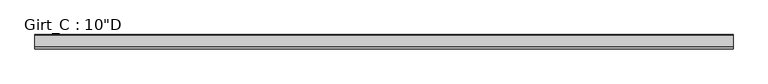
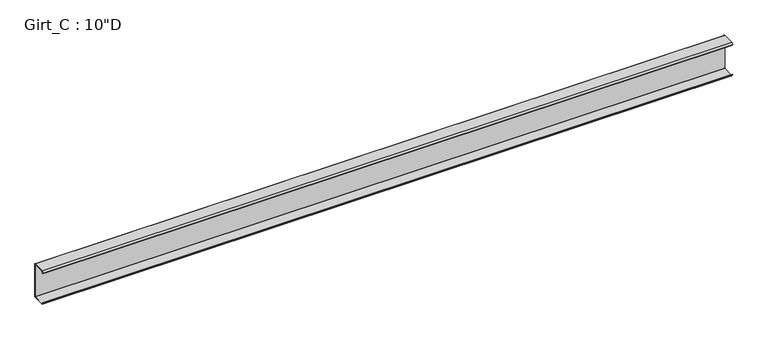
"""IFC4 building model written with IfcOpenShell, lengths in millimetres: beam geometry."""

import ifcopenshell
import ifcopenshell.guid

model = None  # the IFC model being written
_history = None  # IfcOwnerHistory: only IFC2X3 demands one
_inside = {}  # id of a spatial element -> (the spatial element, [elements in it])
_under = {}  # id of a project, library or spatial element -> (it, [spatial elements below it])
_declared = {}  # id of a project -> (the project, [libraries it declares])
_typed = {}  # id of a type object -> (the type object, [elements of that type])
_made_of = {}  # id of a material, layer set ... -> (it, [elements and type objects made of it])


def new_model(schema):
    """Start an empty IFC model of exactly this schema.

    Asked for "IFC4X3", IfcOpenShell would pick the latest addendum, in which some entities
    have other attributes; the version numbers below select the first issue.
    IFC2X3 requires an IfcOwnerHistory on every rooted entity: one is made here for all.
    """
    global model, _history
    if schema == "IFC4X3":
        model = ifcopenshell.file(schema_version=(4, 3, 0, 0))
    else:
        model = ifcopenshell.file(schema=schema)
    _inside.clear()
    _under.clear()
    _declared.clear()
    _typed.clear()
    _made_of.clear()
    _history = None
    if model.schema == "IFC2X3":
        org = make("IfcOrganization", Name="unknown")
        user = make(
            "IfcPersonAndOrganization",
            ThePerson=make("IfcPerson", FamilyName="unknown"),
            TheOrganization=org,
        )
        app = make(
            "IfcApplication",
            ApplicationDeveloper=org,
            Version="unknown",
            ApplicationFullName="unknown",
            ApplicationIdentifier="unknown",
        )
        _history = make(
            "IfcOwnerHistory",
            OwningUser=user,
            OwningApplication=app,
            ChangeAction="ADDED",
            CreationDate=0,
        )
    return model


def make(cls, **values):
    """One entity of the class cls with the attributes given. An attribute that is None is left unset."""
    return model.create_entity(
        cls, **{name: value for name, value in values.items() if value is not None}
    )


def rooted(cls, **values):
    """An entity with a GlobalId (a new one), such as an element, a storey or a relation."""
    return make(cls, GlobalId=ifcopenshell.guid.new(), OwnerHistory=_history, **values)


def si_unit(unit_type, name, prefix=None):
    """IfcSIUnit, for example si_unit("LENGTHUNIT", "METRE", prefix="MILLI")."""
    return make("IfcSIUnit", UnitType=unit_type, Prefix=prefix, Name=name)


def assignment(units):
    """IfcUnitAssignment: the units of a project."""
    return None if units is None else make("IfcUnitAssignment", Units=units)


def point(xyz):
    """IfcCartesianPoint."""
    return None if xyz is None else make("IfcCartesianPoint", Coordinates=xyz)


def direction(xyz):
    """IfcDirection."""
    return None if xyz is None else make("IfcDirection", DirectionRatios=xyz)


def frame(location, z_axis=None, x_axis=None):
    """IfcAxis2Placement3D, a coordinate frame: its origin and axes. An axis left out is left unset."""
    return make(
        "IfcAxis2Placement3D",
        Location=point(location),
        Axis=direction(z_axis),
        RefDirection=direction(x_axis),
    )


def frame_2d(location, x_axis=None):
    """IfcAxis2Placement2D, a coordinate frame in the plane: its origin and x axis."""
    return make(
        "IfcAxis2Placement2D", Location=point(location), RefDirection=direction(x_axis)
    )


def origin():
    """The frame at (0, 0, 0) with its axes left unset."""
    return frame((0.0, 0.0, 0.0))


def place(relative_to, where):
    """IfcLocalPlacement: puts the frame where relative to a parent placement (None: the world)."""
    return make(
        "IfcLocalPlacement", PlacementRelTo=relative_to, RelativePlacement=where
    )


def context(
    kind, dimensions, precision=None, world=None, true_north=None, identifier=None
):
    """IfcGeometricRepresentationContext, for example the 3D "Model" context."""
    return make(
        "IfcGeometricRepresentationContext",
        ContextIdentifier=identifier,
        ContextType=kind,
        CoordinateSpaceDimension=dimensions,
        Precision=precision,
        WorldCoordinateSystem=world,
        TrueNorth=true_north,
    )


def project(units=None, contexts=None):
    """IfcProject with its units and contexts."""
    return rooted(
        "IfcProject",
        Name="project",
        RepresentationContexts=contexts,
        UnitsInContext=assignment(units),
    )


def spatial(cls, under=None, at=None, **own):
    """A site, building, storey or space (cls), placed at a placement, below another one or the project."""
    s = rooted(cls, ObjectPlacement=at, **own)
    if under is not None:
        _under.setdefault(under.id(), (under, []))[1].append(s)
    return s


def polyline(points):
    """IfcPolyline through the points."""
    return make("IfcPolyline", Points=[point(p) for p in points])


def circle_curve(where, radius):
    """IfcCircle in the frame where."""
    return make("IfcCircle", Position=where, Radius=radius)


def trimmed(basis, trim1, trim2, sense, master):
    """IfcTrimmedCurve: the piece of a basis curve between two trims."""
    return make(
        "IfcTrimmedCurve",
        BasisCurve=basis,
        Trim1=trim1,
        Trim2=trim2,
        SenseAgreement=sense,
        MasterRepresentation=master,
    )


def segment(curve, same_sense, transition):
    """IfcCompositeCurveSegment."""
    return make(
        "IfcCompositeCurveSegment",
        Transition=transition,
        SameSense=same_sense,
        ParentCurve=curve,
    )


def composite_curve(segments, self_intersect=None):
    """IfcCompositeCurve: segments joined end to end."""
    return make("IfcCompositeCurve", Segments=segments, SelfIntersect=self_intersect)


def outline(outer, holes=None, kind="AREA"):
    """IfcArbitraryClosedProfileDef: a profile drawn as a closed curve; with holes, ...WithVoids."""
    if holes is None:
        return make("IfcArbitraryClosedProfileDef", ProfileType=kind, OuterCurve=outer)
    return make(
        "IfcArbitraryProfileDefWithVoids",
        ProfileType=kind,
        OuterCurve=outer,
        InnerCurves=holes,
    )


def extrude(swept, where, along, depth):
    """IfcExtrudedAreaSolid: the profile swept, set in the frame where, extruded along a direction by depth."""
    return make(
        "IfcExtrudedAreaSolid",
        SweptArea=swept,
        Position=where,
        ExtrudedDirection=direction(along),
        Depth=depth,
    )


def shape(context_of_items, identifier, shape_type, items):
    """IfcShapeRepresentation: the items that make up one representation, for example the "Body"."""
    return make(
        "IfcShapeRepresentation",
        ContextOfItems=context_of_items,
        RepresentationIdentifier=identifier,
        RepresentationType=shape_type,
        Items=items,
    )


def source(mapping_origin, context_of_items, identifier, shape_type, items):
    """IfcRepresentationMap: a shape defined once, which mapped items show again and again."""
    return make(
        "IfcRepresentationMap",
        MappingOrigin=mapping_origin,
        MappedRepresentation=shape(context_of_items, identifier, shape_type, items),
    )


def transform(
    local_origin,
    x_axis=None,
    y_axis=None,
    z_axis=None,
    scale=None,
    scale2=None,
    scale3=None,
    uniform=True,
):
    """IfcCartesianTransformationOperator3D, or its non-uniform kind. x_axis, y_axis, z_axis: its Axis1, 2, 3."""
    if uniform:
        return make(
            "IfcCartesianTransformationOperator3D",
            Axis1=direction(x_axis),
            Axis2=direction(y_axis),
            LocalOrigin=point(local_origin),
            Scale=scale,
            Axis3=direction(z_axis),
        )
    return make(
        "IfcCartesianTransformationOperator3DnonUniform",
        Axis1=direction(x_axis),
        Axis2=direction(y_axis),
        LocalOrigin=point(local_origin),
        Scale=scale,
        Axis3=direction(z_axis),
        Scale2=scale2,
        Scale3=scale3,
    )


def mapped(mapping_source, mapping_target):
    """IfcMappedItem: shows the shape of a source again, moved by a transform."""
    return make(
        "IfcMappedItem", MappingSource=mapping_source, MappingTarget=mapping_target
    )


def made_of(thing, what):
    """Note that an element or type object is made of a material, layer set ...; save() writes the relation."""
    if what is not None:
        _made_of.setdefault(what.id(), (what, []))[1].append(thing)
    return thing


def element(
    cls,
    number,
    at=None,
    inside=None,
    cuts=None,
    type_object=None,
    material=None,
    context=None,
    identifier="Body",
    shape_type=None,
    held_by="IfcProductDefinitionShape",
    body=None,
    shapes=None,
    **own,
):
    """One element of the class cls, such as IfcWall. Its Tag is "e" and its number.

    at: its placement. inside: the storey or other place that contains it. cuts: it is an
    opening in that element (IfcRelVoidsElement). A single representation is given by context,
    identifier, shape_type and body (its items); several are given by shapes. held_by: the class
    of the entity that holds the representations. save() writes the other relations.
    """
    e = rooted(cls, Tag="e%d" % number, ObjectPlacement=at, **own)
    if body is not None:
        shapes = [shape(context, identifier, shape_type, body)]
    if shapes is not None:
        e.Representation = make(held_by, Representations=shapes)
    if inside is not None:
        _inside.setdefault(inside.id(), (inside, []))[1].append(e)
    if cuts is not None:
        rooted(
            "IfcRelVoidsElement", RelatingBuildingElement=cuts, RelatedOpeningElement=e
        )
    if type_object is not None:
        _typed.setdefault(type_object.id(), (type_object, []))[1].append(e)
    return made_of(e, material)


def aggregate(whole, parts):
    """IfcRelAggregates: a whole, such as a stair, and the parts it consists of."""
    return rooted("IfcRelAggregates", RelatingObject=whole, RelatedObjects=parts)


def save(model, path):
    """Write the relations noted so far, then the file.

    IfcRelAggregates (storeys below a building ...), IfcRelContainedInSpatialStructure (elements
    in a storey), IfcRelDefinesByType, IfcRelAssociatesMaterial and IfcRelDeclares: one each for
    every whole, place, type object, material and project.
    """
    for whole, parts in _under.values():
        aggregate(whole, parts)
    for where, things in _inside.values():
        rooted(
            "IfcRelContainedInSpatialStructure",
            RelatedElements=things,
            RelatingStructure=where,
        )
    for kind, things in _typed.values():
        rooted("IfcRelDefinesByType", RelatedObjects=things, RelatingType=kind)
    for what, things in _made_of.values():
        rooted("IfcRelAssociatesMaterial", RelatedObjects=things, RelatingMaterial=what)
    for by, libraries in _declared.values():
        rooted("IfcRelDeclares", RelatingContext=by, RelatedDefinitions=libraries)
    model.write(path)


def beam_7096158d(model_context):
    return source(origin(), model_context, "Body", "SweptSolid", [
        extrude(outline(composite_curve([segment(polyline([(-87.5109375, 127.0), (-3.3734375, 127.0)]), True, "CONTINUOUS"), segment(trimmed(circle_curve(frame_2d((-3.3734375, 122.2375)), 4.7625), [point((-3.3734375, 127.0))], [point((1.3890625, 122.2375))], False, "CARTESIAN"), True, "CONTINUOUS"), segment(polyline([(1.3890625, 122.2375), (1.3890625, -122.2375)]), True, "CONTINUOUS"), segment(trimmed(circle_curve(frame_2d((-3.3734375, -122.2375)), 4.7625), [point((1.3890625, -122.2375))], [point((-3.3734375, -127.0))], False, "CARTESIAN"), True, "CONTINUOUS"), segment(polyline([(-3.3734375, -127.0), (-87.5109375, -127.0), (-99.7792647, -112.379177), (-97.6510975, -110.5934327), (-86.2154765, -124.221875), (-3.2694106, -124.221875)]), True, "CONTINUOUS"), segment(trimmed(circle_curve(frame_2d((-3.3748024, -122.2389339)), 1.9857399), [point((-3.2694106, -124.221875))], [point((-1.3890625, -122.2389339))], True, "CARTESIAN"), True, "CONTINUOUS"), segment(polyline([(-1.3890625, -122.2389339), (-1.3890625, 122.2381931)]), True, "CONTINUOUS"), segment(trimmed(circle_curve(frame_2d((-3.3741066, 122.2381931)), 1.9850441), [point((-1.3890625, 122.2381931))], [point((-3.3005807, 124.221875))], True, "CARTESIAN"), True, "CONTINUOUS"), segment(polyline([(-3.3005807, 124.221875), (-86.2154765, 124.221875), (-97.6278742, 110.621109), (-99.7560415, 112.4068534), (-87.5109375, 127.0)]), True, "CONTINUOUS")], self_intersect=False)), frame((-2501.6206, 0.0, 0.0), z_axis=(1.0, 0.0, 0.0), x_axis=(0.0, 1.0, 0.0)), (0.0, 0.0, 1.0), 4939.538),
    ])


if __name__ == "__main__":
    model = new_model("IFC4")
    model_context = context("Model", 3, world=origin())
    ifc_project = project(units=[si_unit("LENGTHUNIT", "METRE", prefix="MILLI")], contexts=[model_context])
    site = spatial("IfcSite", under=ifc_project)
    building = spatial("IfcBuilding", under=site)
    placement = place(None, origin())
    beam_shape = beam_7096158d(model_context)
    element("IfcBeam", 1, ObjectType="Girt_C : 10\"D", at=placement, inside=building, context=model_context, shape_type="MappedRepresentation", body=[
        mapped(beam_shape, transform((0.0, 0.0, 0.0), x_axis=(1.0, 0.0, 0.0), y_axis=(0.0, 1.0, 0.0), z_axis=(0.0, 0.0, 1.0))),
    ])
    save(model, "model.ifc")

# Revit data of these elements
# Type "Girt_C : 10\"D"
#   half leg = 0' - 1 3/4"
#   Web_Thickness = 0' - 0 7/64"
#   Length [instance default] = 10' - 0"
#   Leg_1 = 0' - 3 1/2"
#   Height = 0' - 10"
#   Structural Material [instance default] = none
# Element 1 (IfcBeam, "Girt_C : 10\"D")
#   Structural Material = STRUCTURAL STEEL - SEE STRUCT. DWGS
#   Materials on its faces: "STRUCTURAL STEEL - SEE STRUCT. DWGS"
# Materials
#   "STRUCTURAL STEEL - SEE STRUCT. DWGS": class "Metal", colour RGB 137 146 153, transparency 0, Description = "Steel, mill finish", Cost = 0
